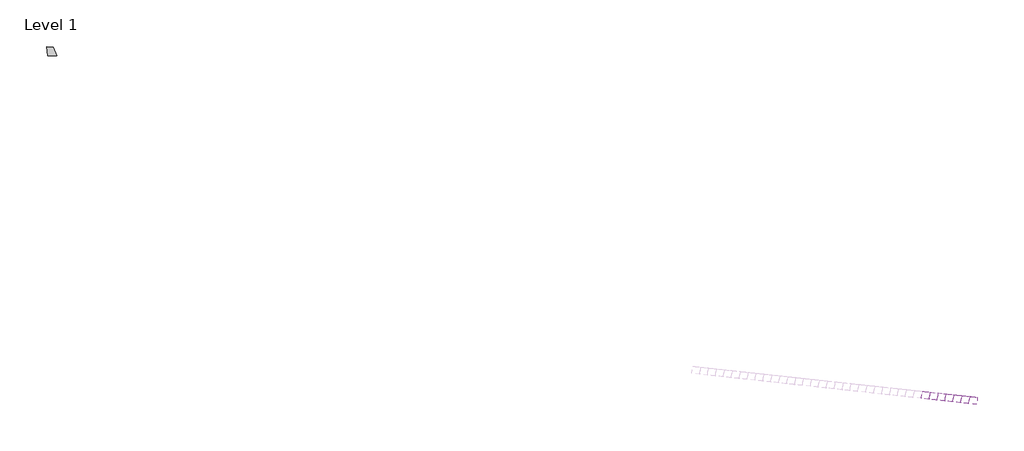
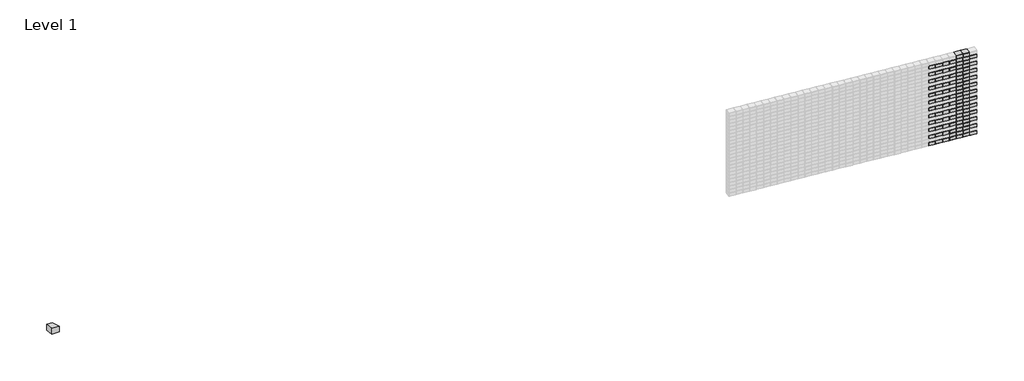
# One storey, part 18 of 18: 111 proxies.
"""IFC4 building model written with IfcOpenShell, lengths in millimetres."""

import ifcopenshell
import ifcopenshell.guid

model = None  # the IFC model being written
_history = None  # IfcOwnerHistory: only IFC2X3 demands one
_inside = {}  # id of a spatial element -> (the spatial element, [elements in it])
_under = {}  # id of a project, library or spatial element -> (it, [spatial elements below it])
_declared = {}  # id of a project -> (the project, [libraries it declares])
_typed = {}  # id of a type object -> (the type object, [elements of that type])
_made_of = {}  # id of a material, layer set ... -> (it, [elements and type objects made of it])


def new_model(schema):
    """Start an empty IFC model of exactly this schema.

    Asked for "IFC4X3", IfcOpenShell would pick the latest addendum, in which some entities
    have other attributes; the version numbers below select the first issue.
    IFC2X3 requires an IfcOwnerHistory on every rooted entity: one is made here for all.
    """
    global model, _history
    if schema == "IFC4X3":
        model = ifcopenshell.file(schema_version=(4, 3, 0, 0))
    else:
        model = ifcopenshell.file(schema=schema)
    _inside.clear()
    _under.clear()
    _declared.clear()
    _typed.clear()
    _made_of.clear()
    _history = None
    if model.schema == "IFC2X3":
        org = make("IfcOrganization", Name="unknown")
        user = make(
            "IfcPersonAndOrganization",
            ThePerson=make("IfcPerson", FamilyName="unknown"),
            TheOrganization=org,
        )
        app = make(
            "IfcApplication",
            ApplicationDeveloper=org,
            Version="unknown",
            ApplicationFullName="unknown",
            ApplicationIdentifier="unknown",
        )
        _history = make(
            "IfcOwnerHistory",
            OwningUser=user,
            OwningApplication=app,
            ChangeAction="ADDED",
            CreationDate=0,
        )
    return model


def make(cls, **values):
    """One entity of the class cls with the attributes given. An attribute that is None is left unset."""
    return model.create_entity(
        cls, **{name: value for name, value in values.items() if value is not None}
    )


def rooted(cls, **values):
    """An entity with a GlobalId (a new one), such as an element, a storey or a relation."""
    return make(cls, GlobalId=ifcopenshell.guid.new(), OwnerHistory=_history, **values)


def si_unit(unit_type, name, prefix=None):
    """IfcSIUnit, for example si_unit("LENGTHUNIT", "METRE", prefix="MILLI")."""
    return make("IfcSIUnit", UnitType=unit_type, Prefix=prefix, Name=name)


def assignment(units):
    """IfcUnitAssignment: the units of a project."""
    return None if units is None else make("IfcUnitAssignment", Units=units)


def point(xyz):
    """IfcCartesianPoint."""
    return None if xyz is None else make("IfcCartesianPoint", Coordinates=xyz)


def direction(xyz):
    """IfcDirection."""
    return None if xyz is None else make("IfcDirection", DirectionRatios=xyz)


def frame(location, z_axis=None, x_axis=None):
    """IfcAxis2Placement3D, a coordinate frame: its origin and axes. An axis left out is left unset."""
    return make(
        "IfcAxis2Placement3D",
        Location=point(location),
        Axis=direction(z_axis),
        RefDirection=direction(x_axis),
    )


def origin():
    """The frame at (0, 0, 0) with its axes left unset."""
    return frame((0.0, 0.0, 0.0))


def origin_with_axes():
    """The frame at (0, 0, 0) with the z axis (0, 0, 1) and the x axis (1, 0, 0) written out."""
    return frame((0.0, 0.0, 0.0), z_axis=(0.0, 0.0, 1.0), x_axis=(1.0, 0.0, 0.0))


def place(relative_to, where):
    """IfcLocalPlacement: puts the frame where relative to a parent placement (None: the world)."""
    return make(
        "IfcLocalPlacement", PlacementRelTo=relative_to, RelativePlacement=where
    )


def context(
    kind, dimensions, precision=None, world=None, true_north=None, identifier=None
):
    """IfcGeometricRepresentationContext, for example the 3D "Model" context."""
    return make(
        "IfcGeometricRepresentationContext",
        ContextIdentifier=identifier,
        ContextType=kind,
        CoordinateSpaceDimension=dimensions,
        Precision=precision,
        WorldCoordinateSystem=world,
        TrueNorth=true_north,
    )


def project(units=None, contexts=None):
    """IfcProject with its units and contexts."""
    return rooted(
        "IfcProject",
        Name="project",
        RepresentationContexts=contexts,
        UnitsInContext=assignment(units),
    )


def spatial(cls, under=None, at=None, **own):
    """A site, building, storey or space (cls), placed at a placement, below another one or the project."""
    s = rooted(cls, ObjectPlacement=at, **own)
    if under is not None:
        _under.setdefault(under.id(), (under, []))[1].append(s)
    return s


def polyline(points):
    """IfcPolyline through the points."""
    return make("IfcPolyline", Points=[point(p) for p in points])


def outline(outer, holes=None, kind="AREA"):
    """IfcArbitraryClosedProfileDef: a profile drawn as a closed curve; with holes, ...WithVoids."""
    if holes is None:
        return make("IfcArbitraryClosedProfileDef", ProfileType=kind, OuterCurve=outer)
    return make(
        "IfcArbitraryProfileDefWithVoids",
        ProfileType=kind,
        OuterCurve=outer,
        InnerCurves=holes,
    )


def extrude(swept, where, along, depth):
    """IfcExtrudedAreaSolid: the profile swept, set in the frame where, extruded along a direction by depth."""
    return make(
        "IfcExtrudedAreaSolid",
        SweptArea=swept,
        Position=where,
        ExtrudedDirection=direction(along),
        Depth=depth,
    )


def shape(context_of_items, identifier, shape_type, items):
    """IfcShapeRepresentation: the items that make up one representation, for example the "Body"."""
    return make(
        "IfcShapeRepresentation",
        ContextOfItems=context_of_items,
        RepresentationIdentifier=identifier,
        RepresentationType=shape_type,
        Items=items,
    )


def source(mapping_origin, context_of_items, identifier, shape_type, items):
    """IfcRepresentationMap: a shape defined once, which mapped items show again and again."""
    return make(
        "IfcRepresentationMap",
        MappingOrigin=mapping_origin,
        MappedRepresentation=shape(context_of_items, identifier, shape_type, items),
    )


def transform(
    local_origin,
    x_axis=None,
    y_axis=None,
    z_axis=None,
    scale=None,
    scale2=None,
    scale3=None,
    uniform=True,
):
    """IfcCartesianTransformationOperator3D, or its non-uniform kind. x_axis, y_axis, z_axis: its Axis1, 2, 3."""
    if uniform:
        return make(
            "IfcCartesianTransformationOperator3D",
            Axis1=direction(x_axis),
            Axis2=direction(y_axis),
            LocalOrigin=point(local_origin),
            Scale=scale,
            Axis3=direction(z_axis),
        )
    return make(
        "IfcCartesianTransformationOperator3DnonUniform",
        Axis1=direction(x_axis),
        Axis2=direction(y_axis),
        LocalOrigin=point(local_origin),
        Scale=scale,
        Axis3=direction(z_axis),
        Scale2=scale2,
        Scale3=scale3,
    )


def mapped(mapping_source, mapping_target):
    """IfcMappedItem: shows the shape of a source again, moved by a transform."""
    return make(
        "IfcMappedItem", MappingSource=mapping_source, MappingTarget=mapping_target
    )


def made_of(thing, what):
    """Note that an element or type object is made of a material, layer set ...; save() writes the relation."""
    if what is not None:
        _made_of.setdefault(what.id(), (what, []))[1].append(thing)
    return thing


def element(
    cls,
    number,
    at=None,
    inside=None,
    cuts=None,
    type_object=None,
    material=None,
    context=None,
    identifier="Body",
    shape_type=None,
    held_by="IfcProductDefinitionShape",
    body=None,
    shapes=None,
    **own,
):
    """One element of the class cls, such as IfcWall. Its Tag is "e" and its number.

    at: its placement. inside: the storey or other place that contains it. cuts: it is an
    opening in that element (IfcRelVoidsElement). A single representation is given by context,
    identifier, shape_type and body (its items); several are given by shapes. held_by: the class
    of the entity that holds the representations. save() writes the other relations.
    """
    e = rooted(cls, Tag="e%d" % number, ObjectPlacement=at, **own)
    if body is not None:
        shapes = [shape(context, identifier, shape_type, body)]
    if shapes is not None:
        e.Representation = make(held_by, Representations=shapes)
    if inside is not None:
        _inside.setdefault(inside.id(), (inside, []))[1].append(e)
    if cuts is not None:
        rooted(
            "IfcRelVoidsElement", RelatingBuildingElement=cuts, RelatedOpeningElement=e
        )
    if type_object is not None:
        _typed.setdefault(type_object.id(), (type_object, []))[1].append(e)
    return made_of(e, material)


def aggregate(whole, parts):
    """IfcRelAggregates: a whole, such as a stair, and the parts it consists of."""
    return rooted("IfcRelAggregates", RelatingObject=whole, RelatedObjects=parts)


def save(model, path):
    """Write the relations noted so far, then the file.

    IfcRelAggregates (storeys below a building ...), IfcRelContainedInSpatialStructure (elements
    in a storey), IfcRelDefinesByType, IfcRelAssociatesMaterial and IfcRelDeclares: one each for
    every whole, place, type object, material and project.
    """
    for whole, parts in _under.values():
        aggregate(whole, parts)
    for where, things in _inside.values():
        rooted(
            "IfcRelContainedInSpatialStructure",
            RelatedElements=things,
            RelatingStructure=where,
        )
    for kind, things in _typed.values():
        rooted("IfcRelDefinesByType", RelatedObjects=things, RelatingType=kind)
    for what, things in _made_of.values():
        rooted("IfcRelAssociatesMaterial", RelatedObjects=things, RelatingMaterial=what)
    for by, libraries in _declared.values():
        rooted("IfcRelDeclares", RelatingContext=by, RelatedDefinitions=libraries)
    model.write(path)


def geel_a5fc7152(model_context):
    return source(origin(), model_context, "Body", "SweptSolid", [
        extrude(outline(polyline([(131.1871262, 51.8695461), (24.8461542, 24.0369432), (23.5801491, 28.8740117), (125.0840527, 55.4406095), (111.9430518, 105.6488784), (10.4391482, 79.0822806), (9.1731432, 83.919349), (115.5141152, 111.7519519), (131.1871262, 51.8695461)])), origin_with_axes(), (0.0, 0.0, 1.0), 95.0),
        extrude(outline(polyline([(111.9430518, 105.6488784), (125.0840527, 55.4406095), (23.5801491, 28.8740117), (10.4391482, 79.0822806), (111.9430518, 105.6488784)])), origin_with_axes(), (0.0, 0.0, 1.0), 100.0),
    ])


def geel_ff5a4212(model_context):
    return source(origin(), model_context, "Body", "SweptSolid", [
        extrude(outline(polyline([(24.8461542, 24.0369432), (9.1731432, 83.919349), (115.5141152, 111.7519519), (116.7801202, 106.9148835), (15.2762167, 80.3482856), (28.4172176, 30.1400167), (129.9211211, 56.7066146), (131.1871262, 51.8695461), (24.8461542, 24.0369432)])), origin_with_axes(), (0.0, 0.0, 1.0), 95.0),
        extrude(outline(polyline([(116.7801202, 106.9148835), (129.9211211, 56.7066146), (28.4172176, 30.1400167), (15.2762167, 80.3482856), (116.7801202, 106.9148835)])), origin_with_axes(), (0.0, 0.0, 1.0), 100.0),
    ])


def rood_14a66368(model_context):
    return source(origin(), model_context, "Body", "SweptSolid", [
        extrude(outline(polyline([(24.8461542, 24.0369432), (9.1731432, 83.919349), (115.5141152, 111.7519519), (131.1871262, 51.8695461), (24.8461542, 24.0369432)]), holes=[polyline([(125.0840527, 55.4406095), (111.9430518, 105.6488784), (15.2762167, 80.3482856), (28.4172176, 30.1400167), (125.0840527, 55.4406095)])]), origin_with_axes(), (0.0, 0.0, 1.0), 95.0),
        extrude(outline(polyline([(111.9430518, 105.6488784), (125.0840527, 55.4406095), (28.4172176, 30.1400167), (15.2762167, 80.3482856), (111.9430518, 105.6488784)])), origin_with_axes(), (0.0, 0.0, 1.0), 100.0),
    ])


def rood_2ddd8018(model_context):
    return source(origin(), model_context, "Body", "SweptSolid", [
        extrude(outline(polyline([(24.8461542, 24.0369432), (9.1731432, 83.919349), (115.5141152, 111.7519519), (131.1871262, 51.8695461), (126.3500577, 50.6035411), (111.9430518, 105.6488784), (15.2762167, 80.3482856), (29.6832226, 25.3029482), (24.8461542, 24.0369432)])), origin_with_axes(), (0.0, 0.0, 1.0), 95.0),
        extrude(outline(polyline([(111.9430518, 105.6488784), (126.3500577, 50.6035411), (29.6832226, 25.3029482), (15.2762167, 80.3482856), (111.9430518, 105.6488784)])), origin_with_axes(), (0.0, 0.0, 1.0), 100.0),
    ])


def steen_standaard_rood_a5b9f397(model_context):
    return source(origin(), model_context, "Body", "SweptSolid", [
        extrude(outline(polyline([(82.4636514, 127.1543377), (128.4615135, 4.6891223), (4.3616271, 4.9486265), (-12.4180967, 134.7857038), (82.4636514, 127.1543377)])), origin_with_axes(), (0.0, 0.0, 1.0), 100.0),
    ])


model = new_model("IFC4")

# Units and contexts
model_context = context("Model", 3, world=origin())
ifc_project = project(units=[si_unit("LENGTHUNIT", "METRE", prefix="MILLI")], contexts=[model_context])

# Site, building, storey
site = spatial("IfcSite", under=ifc_project)
building = spatial("IfcBuilding", under=site)
storey = spatial("IfcBuildingStorey", under=building, Name="Level 1", Elevation=0.0)

# Proxies
placement = place(None, origin())
geel_shape = geel_a5fc7152(model_context)
element("IfcBuildingElementProxy", 1, Name="Geel", ObjectType="Geel", at=placement, inside=storey, context=model_context, shape_type="MappedRepresentation", body=[
    mapped(geel_shape, transform((12373.9492488, -4657.0823366, 2044.9368847), x_axis=(0.961727550372943, -0.10473475661477032, -0.25320100633785686), y_axis=(0.25171277368867245, -0.02741220845642687, 0.9674136914420308), z_axis=(-0.10826263628608798, -0.9941223272738553, 0.0))),
])
element("IfcBuildingElementProxy", 2, Name="Geel", ObjectType="Geel", at=placement, inside=storey, context=model_context, shape_type="MappedRepresentation", body=[
    mapped(geel_shape, transform((12592.5029772, -4680.8834345, 2168.7358475), x_axis=(0.9617275503729374, -0.1047347566147725, -0.25320100633787673), y_axis=(0.25171277368869216, -0.02741220845642974, 0.9674136914420255), z_axis=(-0.10826263628609081, -0.9941223272738551, 0.0))),
])
element("IfcBuildingElementProxy", 3, Name="Geel", ObjectType="Geel", at=placement, inside=storey, context=model_context, shape_type="MappedRepresentation", body=[
    mapped(geel_shape, transform((12592.5029772, -4680.8834345, 2292.5348104), x_axis=(0.9617275503729374, -0.1047347566147725, -0.25320100633787673), y_axis=(0.25171277368869216, -0.02741220845642974, 0.9674136914420255), z_axis=(-0.10826263628609081, -0.9941223272738551, 0.0))),
])
element("IfcBuildingElementProxy", 4, Name="Geel", ObjectType="Geel", at=placement, inside=storey, context=model_context, shape_type="MappedRepresentation", body=[
    mapped(geel_shape, transform((12592.5029772, -4680.8834345, 2416.3337732), x_axis=(0.9617275503729384, -0.1047347566147726, -0.25320100633787307), y_axis=(0.25171277368868855, -0.02741220845642934, 0.9674136914420265), z_axis=(-0.10826263628609081, -0.994122327273855, 0.0))),
])
element("IfcBuildingElementProxy", 5, Name="Geel", ObjectType="Geel", at=placement, inside=storey, context=model_context, shape_type="MappedRepresentation", body=[
    mapped(geel_shape, transform((12592.5029772, -4680.8834345, 2540.132736), x_axis=(0.9617275503729374, -0.1047347566147725, -0.25320100633787673), y_axis=(0.25171277368869216, -0.02741220845642974, 0.9674136914420255), z_axis=(-0.10826263628609081, -0.9941223272738551, 0.0))),
])
element("IfcBuildingElementProxy", 6, Name="Geel", ObjectType="Geel", at=placement, inside=storey, context=model_context, shape_type="MappedRepresentation", body=[
    mapped(geel_shape, transform((12592.5029772, -4680.8834345, 2663.9316989), x_axis=(0.9617275503729374, -0.1047347566147725, -0.25320100633787673), y_axis=(0.25171277368869216, -0.02741220845642974, 0.9674136914420255), z_axis=(-0.10826263628609081, -0.9941223272738551, 0.0))),
])
element("IfcBuildingElementProxy", 7, Name="Geel", ObjectType="Geel", at=placement, inside=storey, context=model_context, shape_type="MappedRepresentation", body=[
    mapped(geel_shape, transform((12592.5029772, -4680.8834345, 2787.7306617), x_axis=(0.9617275503729374, -0.1047347566147725, -0.25320100633787673), y_axis=(0.25171277368869216, -0.02741220845642974, 0.9674136914420255), z_axis=(-0.10826263628609081, -0.9941223272738551, 0.0))),
])
element("IfcBuildingElementProxy", 8, Name="Geel", ObjectType="Geel", at=placement, inside=storey, context=model_context, shape_type="MappedRepresentation", body=[
    mapped(geel_shape, transform((12592.5029772, -4680.8834345, 2911.5296245), x_axis=(0.9617275503729374, -0.1047347566147725, -0.25320100633787673), y_axis=(0.25171277368869216, -0.02741220845642974, 0.9674136914420255), z_axis=(-0.10826263628609081, -0.9941223272738551, 0.0))),
])
element("IfcBuildingElementProxy", 9, Name="Geel", ObjectType="Geel", at=placement, inside=storey, context=model_context, shape_type="MappedRepresentation", body=[
    mapped(geel_shape, transform((12592.5029772, -4680.8834345, 3035.3285874), x_axis=(0.9617275503729374, -0.1047347566147725, -0.25320100633787673), y_axis=(0.25171277368869216, -0.02741220845642974, 0.9674136914420255), z_axis=(-0.10826263628609081, -0.9941223272738551, 0.0))),
])
element("IfcBuildingElementProxy", 10, Name="Geel", ObjectType="Geel", at=placement, inside=storey, context=model_context, shape_type="MappedRepresentation", body=[
    mapped(geel_shape, transform((12592.5029772, -4680.8834345, 3159.1275502), x_axis=(0.9617275503729374, -0.1047347566147725, -0.25320100633787673), y_axis=(0.25171277368869216, -0.02741220845642974, 0.9674136914420255), z_axis=(-0.10826263628609081, -0.9941223272738551, 0.0))),
])
element("IfcBuildingElementProxy", 11, Name="Geel", ObjectType="Geel", at=placement, inside=storey, context=model_context, shape_type="MappedRepresentation", body=[
    mapped(geel_shape, transform((12592.5029772, -4680.8834345, 3282.926513), x_axis=(0.9617275503729374, -0.1047347566147725, -0.25320100633787673), y_axis=(0.25171277368869216, -0.02741220845642974, 0.9674136914420255), z_axis=(-0.10826263628609081, -0.9941223272738551, 0.0))),
])
element("IfcBuildingElementProxy", 12, Name="Geel", ObjectType="Geel", at=placement, inside=storey, context=model_context, shape_type="MappedRepresentation", body=[
    mapped(geel_shape, transform((12592.5029772, -4680.8834345, 3406.7254759), x_axis=(0.9617275503729374, -0.1047347566147725, -0.25320100633787673), y_axis=(0.25171277368869216, -0.02741220845642974, 0.9674136914420255), z_axis=(-0.10826263628609081, -0.9941223272738551, 0.0))),
])
element("IfcBuildingElementProxy", 13, Name="Geel", ObjectType="Geel", at=placement, inside=storey, context=model_context, shape_type="MappedRepresentation", body=[
    mapped(geel_shape, transform((12592.5029772, -4680.8834345, 2044.9368847), x_axis=(0.9617275503729384, -0.1047347566147726, -0.25320100633787307), y_axis=(0.25171277368868855, -0.02741220845642934, 0.9674136914420265), z_axis=(-0.10826263628609081, -0.994122327273855, 0.0))),
])
geel_2_shape = geel_ff5a4212(model_context)
element("IfcBuildingElementProxy", 14, Name="Geel", ObjectType="Geel", at=placement, inside=storey, context=model_context, shape_type="MappedRepresentation", body=[
    mapped(geel_2_shape, transform((12483.226113, -4668.9828856, 2168.7358475), x_axis=(0.9617275503729374, -0.1047347566147725, -0.25320100633787673), y_axis=(0.25171277368869216, -0.02741220845642974, 0.9674136914420255), z_axis=(-0.10826263628609081, -0.9941223272738551, 0.0))),
])
element("IfcBuildingElementProxy", 15, Name="Geel", ObjectType="Geel", at=placement, inside=storey, context=model_context, shape_type="MappedRepresentation", body=[
    mapped(geel_2_shape, transform((12483.226113, -4668.9828856, 2292.5348104), x_axis=(0.9617275503729374, -0.1047347566147725, -0.25320100633787673), y_axis=(0.25171277368869216, -0.02741220845642974, 0.9674136914420255), z_axis=(-0.10826263628609081, -0.9941223272738551, 0.0))),
])
element("IfcBuildingElementProxy", 16, Name="Geel", ObjectType="Geel", at=placement, inside=storey, context=model_context, shape_type="MappedRepresentation", body=[
    mapped(geel_2_shape, transform((12483.226113, -4668.9828856, 2416.3337732), x_axis=(0.9617275503729384, -0.1047347566147726, -0.25320100633787307), y_axis=(0.25171277368868855, -0.02741220845642934, 0.9674136914420265), z_axis=(-0.10826263628609081, -0.994122327273855, 0.0))),
])
element("IfcBuildingElementProxy", 17, Name="Geel", ObjectType="Geel", at=placement, inside=storey, context=model_context, shape_type="MappedRepresentation", body=[
    mapped(geel_2_shape, transform((12483.226113, -4668.9828856, 2540.132736), x_axis=(0.9617275503729374, -0.1047347566147725, -0.25320100633787673), y_axis=(0.25171277368869216, -0.02741220845642974, 0.9674136914420255), z_axis=(-0.10826263628609081, -0.9941223272738551, 0.0))),
])
element("IfcBuildingElementProxy", 18, Name="Geel", ObjectType="Geel", at=placement, inside=storey, context=model_context, shape_type="MappedRepresentation", body=[
    mapped(geel_2_shape, transform((12483.226113, -4668.9828856, 2663.9316989), x_axis=(0.9617275503729374, -0.1047347566147725, -0.25320100633787673), y_axis=(0.25171277368869216, -0.02741220845642974, 0.9674136914420255), z_axis=(-0.10826263628609081, -0.9941223272738551, 0.0))),
])
element("IfcBuildingElementProxy", 19, Name="Geel", ObjectType="Geel", at=placement, inside=storey, context=model_context, shape_type="MappedRepresentation", body=[
    mapped(geel_2_shape, transform((12483.226113, -4668.9828856, 2787.7306617), x_axis=(0.9617275503729374, -0.1047347566147725, -0.25320100633787673), y_axis=(0.25171277368869216, -0.02741220845642974, 0.9674136914420255), z_axis=(-0.10826263628609081, -0.9941223272738551, 0.0))),
])
element("IfcBuildingElementProxy", 20, Name="Geel", ObjectType="Geel", at=placement, inside=storey, context=model_context, shape_type="MappedRepresentation", body=[
    mapped(geel_2_shape, transform((12483.226113, -4668.9828856, 2911.5296245), x_axis=(0.9617275503729374, -0.1047347566147725, -0.25320100633787673), y_axis=(0.25171277368869216, -0.02741220845642974, 0.9674136914420255), z_axis=(-0.10826263628609081, -0.9941223272738551, 0.0))),
])
element("IfcBuildingElementProxy", 21, Name="Geel", ObjectType="Geel", at=placement, inside=storey, context=model_context, shape_type="MappedRepresentation", body=[
    mapped(geel_2_shape, transform((12483.226113, -4668.9828856, 3035.3285874), x_axis=(0.9617275503729374, -0.1047347566147725, -0.25320100633787673), y_axis=(0.25171277368869216, -0.02741220845642974, 0.9674136914420255), z_axis=(-0.10826263628609081, -0.9941223272738551, 0.0))),
])
element("IfcBuildingElementProxy", 22, Name="Geel", ObjectType="Geel", at=placement, inside=storey, context=model_context, shape_type="MappedRepresentation", body=[
    mapped(geel_2_shape, transform((12483.226113, -4668.9828856, 3159.1275502), x_axis=(0.9617275503729374, -0.1047347566147725, -0.25320100633787673), y_axis=(0.25171277368869216, -0.02741220845642974, 0.9674136914420255), z_axis=(-0.10826263628609081, -0.9941223272738551, 0.0))),
])
element("IfcBuildingElementProxy", 23, Name="Geel", ObjectType="Geel", at=placement, inside=storey, context=model_context, shape_type="MappedRepresentation", body=[
    mapped(geel_2_shape, transform((12483.226113, -4668.9828856, 3282.926513), x_axis=(0.9617275503729374, -0.1047347566147725, -0.25320100633787673), y_axis=(0.25171277368869216, -0.02741220845642974, 0.9674136914420255), z_axis=(-0.10826263628609081, -0.9941223272738551, 0.0))),
])
element("IfcBuildingElementProxy", 24, Name="Geel", ObjectType="Geel", at=placement, inside=storey, context=model_context, shape_type="MappedRepresentation", body=[
    mapped(geel_2_shape, transform((12483.226113, -4668.9828856, 3406.7254759), x_axis=(0.9617275503729374, -0.1047347566147725, -0.25320100633787673), y_axis=(0.25171277368869216, -0.02741220845642974, 0.9674136914420255), z_axis=(-0.10826263628609081, -0.9941223272738551, 0.0))),
])
element("IfcBuildingElementProxy", 25, Name="Geel", ObjectType="Geel", at=placement, inside=storey, context=model_context, shape_type="MappedRepresentation", body=[
    mapped(geel_2_shape, transform((12483.226113, -4668.9828856, 2044.9368847), x_axis=(0.9617275503729384, -0.1047347566147726, -0.25320100633787307), y_axis=(0.25171277368868855, -0.02741220845642934, 0.9674136914420265), z_axis=(-0.10826263628609081, -0.994122327273855, 0.0))),
])
element("IfcBuildingElementProxy", 26, Name="Rood", ObjectType="Rood", at=placement, inside=storey, context=model_context, shape_type="MappedRepresentation", body=[
    mapped(geel_shape, transform((12701.7798414, -4692.7839834, 2106.8363661), x_axis=(0.9617275503729374, -0.1047347566147725, -0.25320100633787673), y_axis=(0.25171277368869216, -0.02741220845642974, 0.9674136914420255), z_axis=(-0.10826263628609081, -0.9941223272738551, 0.0))),
])
element("IfcBuildingElementProxy", 27, Name="Rood", ObjectType="Rood", at=placement, inside=storey, context=model_context, shape_type="MappedRepresentation", body=[
    mapped(geel_shape, transform((12701.7798414, -4692.7839834, 2230.6353289), x_axis=(0.9617275503729384, -0.1047347566147726, -0.25320100633787307), y_axis=(0.25171277368868855, -0.02741220845642934, 0.9674136914420265), z_axis=(-0.10826263628609081, -0.994122327273855, 0.0))),
])
element("IfcBuildingElementProxy", 28, Name="Rood", ObjectType="Rood", at=placement, inside=storey, context=model_context, shape_type="MappedRepresentation", body=[
    mapped(geel_shape, transform((12701.7798414, -4692.7839834, 2354.4342918), x_axis=(0.9617275503729374, -0.1047347566147725, -0.25320100633787673), y_axis=(0.25171277368869216, -0.02741220845642974, 0.9674136914420255), z_axis=(-0.10826263628609081, -0.9941223272738551, 0.0))),
])
element("IfcBuildingElementProxy", 29, Name="Rood", ObjectType="Rood", at=placement, inside=storey, context=model_context, shape_type="MappedRepresentation", body=[
    mapped(geel_shape, transform((12701.7798414, -4692.7839834, 2478.2332546), x_axis=(0.9617275503729374, -0.1047347566147725, -0.25320100633787673), y_axis=(0.25171277368869216, -0.02741220845642974, 0.9674136914420255), z_axis=(-0.10826263628609081, -0.9941223272738551, 0.0))),
])
element("IfcBuildingElementProxy", 30, Name="Rood", ObjectType="Rood", at=placement, inside=storey, context=model_context, shape_type="MappedRepresentation", body=[
    mapped(geel_shape, transform((12701.7798414, -4692.7839834, 2602.0322174), x_axis=(0.9617275503729394, -0.10473475661477268, -0.2532010063378695), y_axis=(0.2517127736886849, -0.027412208456428923, 0.9674136914420275), z_axis=(-0.1082626362860908, -0.9941223272738551, 0.0))),
])
element("IfcBuildingElementProxy", 31, Name="Rood", ObjectType="Rood", at=placement, inside=storey, context=model_context, shape_type="MappedRepresentation", body=[
    mapped(geel_shape, transform((12701.7798414, -4692.7839834, 2725.8311803), x_axis=(0.9617275503729374, -0.1047347566147725, -0.25320100633787673), y_axis=(0.25171277368869216, -0.02741220845642974, 0.9674136914420255), z_axis=(-0.10826263628609081, -0.9941223272738551, 0.0))),
])
element("IfcBuildingElementProxy", 32, Name="Rood", ObjectType="Rood", at=placement, inside=storey, context=model_context, shape_type="MappedRepresentation", body=[
    mapped(geel_shape, transform((12701.7798414, -4692.7839834, 2849.6301431), x_axis=(0.9617275503729374, -0.1047347566147725, -0.25320100633787673), y_axis=(0.25171277368869216, -0.02741220845642974, 0.9674136914420255), z_axis=(-0.10826263628609081, -0.9941223272738551, 0.0))),
])
element("IfcBuildingElementProxy", 33, Name="Rood", ObjectType="Rood", at=placement, inside=storey, context=model_context, shape_type="MappedRepresentation", body=[
    mapped(geel_shape, transform((12701.7798414, -4692.7839834, 2973.4291059), x_axis=(0.9617275503729374, -0.1047347566147725, -0.25320100633787673), y_axis=(0.25171277368869216, -0.02741220845642974, 0.9674136914420255), z_axis=(-0.10826263628609081, -0.9941223272738551, 0.0))),
])
element("IfcBuildingElementProxy", 34, Name="Rood", ObjectType="Rood", at=placement, inside=storey, context=model_context, shape_type="MappedRepresentation", body=[
    mapped(geel_shape, transform((12701.7798414, -4692.7839834, 3097.2280688), x_axis=(0.9617275503729394, -0.10473475661477268, -0.2532010063378695), y_axis=(0.2517127736886849, -0.027412208456428923, 0.9674136914420275), z_axis=(-0.1082626362860908, -0.9941223272738551, 0.0))),
])
element("IfcBuildingElementProxy", 35, Name="Rood", ObjectType="Rood", at=placement, inside=storey, context=model_context, shape_type="MappedRepresentation", body=[
    mapped(geel_shape, transform((12701.7798414, -4692.7839834, 3221.0270316), x_axis=(0.9617275503729374, -0.1047347566147725, -0.25320100633787673), y_axis=(0.25171277368869216, -0.02741220845642974, 0.9674136914420255), z_axis=(-0.10826263628609081, -0.9941223272738551, 0.0))),
])
element("IfcBuildingElementProxy", 36, Name="Rood", ObjectType="Rood", at=placement, inside=storey, context=model_context, shape_type="MappedRepresentation", body=[
    mapped(geel_shape, transform((12701.7798414, -4692.7839834, 3344.8259944), x_axis=(0.9617275503729357, -0.10473475661477229, -0.2532010063378841), y_axis=(0.2517127736886993, -0.027412208456430498, 0.9674136914420237), z_axis=(-0.10826263628609081, -0.9941223272738551, 0.0))),
])
element("IfcBuildingElementProxy", 37, Name="Rood", ObjectType="Rood", at=placement, inside=storey, context=model_context, shape_type="MappedRepresentation", body=[
    mapped(geel_shape, transform((12701.7798414, -4692.7839834, 1983.0374033), x_axis=(0.9617275503729374, -0.1047347566147725, -0.25320100633787673), y_axis=(0.25171277368869216, -0.02741220845642974, 0.9674136914420255), z_axis=(-0.10826263628609081, -0.9941223272738551, 0.0))),
])
rood_shape = rood_14a66368(model_context)
element("IfcBuildingElementProxy", 38, Name="Rood", ObjectType="Rood", at=placement, inside=storey, context=model_context, shape_type="MappedRepresentation", body=[
    mapped(rood_shape, transform((12046.1186563, -4621.3806898, 2106.8363661), x_axis=(0.9617275503729374, -0.10473475661477244, -0.25320100633787673), y_axis=(0.25171277368869216, -0.02741220845642972, 0.9674136914420255), z_axis=(-0.10826263628609079, -0.9941223272738551, 0.0))),
])
element("IfcBuildingElementProxy", 39, Name="Rood", ObjectType="Rood", at=placement, inside=storey, context=model_context, shape_type="MappedRepresentation", body=[
    mapped(rood_shape, transform((12046.1186563, -4621.3806898, 2230.6353289), x_axis=(0.9617275503729384, -0.10473475661477256, -0.25320100633787307), y_axis=(0.25171277368868855, -0.02741220845642932, 0.9674136914420265), z_axis=(-0.10826263628609077, -0.994122327273855, 0.0))),
])
element("IfcBuildingElementProxy", 40, Name="Rood", ObjectType="Rood", at=placement, inside=storey, context=model_context, shape_type="MappedRepresentation", body=[
    mapped(rood_shape, transform((12046.1186563, -4621.3806898, 2354.4342918), x_axis=(0.9617275503729374, -0.10473475661477244, -0.25320100633787673), y_axis=(0.25171277368869216, -0.02741220845642972, 0.9674136914420255), z_axis=(-0.10826263628609079, -0.9941223272738551, 0.0))),
])
element("IfcBuildingElementProxy", 41, Name="Rood", ObjectType="Rood", at=placement, inside=storey, context=model_context, shape_type="MappedRepresentation", body=[
    mapped(rood_shape, transform((12046.1186563, -4621.3806898, 2478.2332546), x_axis=(0.9617275503729374, -0.10473475661477244, -0.25320100633787673), y_axis=(0.25171277368869216, -0.02741220845642972, 0.9674136914420255), z_axis=(-0.10826263628609079, -0.9941223272738551, 0.0))),
])
element("IfcBuildingElementProxy", 42, Name="Rood", ObjectType="Rood", at=placement, inside=storey, context=model_context, shape_type="MappedRepresentation", body=[
    mapped(rood_shape, transform((12046.1186563, -4621.3806898, 2602.0322174), x_axis=(0.9617275503729394, -0.10473475661477263, -0.2532010063378695), y_axis=(0.2517127736886849, -0.027412208456428916, 0.9674136914420275), z_axis=(-0.10826263628609077, -0.9941223272738551, 0.0))),
])
element("IfcBuildingElementProxy", 43, Name="Rood", ObjectType="Rood", at=placement, inside=storey, context=model_context, shape_type="MappedRepresentation", body=[
    mapped(rood_shape, transform((12046.1186563, -4621.3806898, 2725.8311803), x_axis=(0.9617275503729374, -0.10473475661477244, -0.25320100633787673), y_axis=(0.25171277368869216, -0.02741220845642972, 0.9674136914420255), z_axis=(-0.10826263628609079, -0.9941223272738551, 0.0))),
])
element("IfcBuildingElementProxy", 44, Name="Rood", ObjectType="Rood", at=placement, inside=storey, context=model_context, shape_type="MappedRepresentation", body=[
    mapped(rood_shape, transform((12046.1186563, -4621.3806898, 2849.6301431), x_axis=(0.9617275503729374, -0.10473475661477244, -0.25320100633787673), y_axis=(0.25171277368869216, -0.02741220845642972, 0.9674136914420255), z_axis=(-0.10826263628609079, -0.9941223272738551, 0.0))),
])
element("IfcBuildingElementProxy", 45, Name="Rood", ObjectType="Rood", at=placement, inside=storey, context=model_context, shape_type="MappedRepresentation", body=[
    mapped(rood_shape, transform((12046.1186563, -4621.3806898, 2973.4291059), x_axis=(0.9617275503729374, -0.10473475661477244, -0.25320100633787673), y_axis=(0.25171277368869216, -0.02741220845642972, 0.9674136914420255), z_axis=(-0.10826263628609079, -0.9941223272738551, 0.0))),
])
element("IfcBuildingElementProxy", 46, Name="Rood", ObjectType="Rood", at=placement, inside=storey, context=model_context, shape_type="MappedRepresentation", body=[
    mapped(rood_shape, transform((12046.1186563, -4621.3806898, 3097.2280688), x_axis=(0.9617275503729394, -0.10473475661477263, -0.2532010063378695), y_axis=(0.2517127736886849, -0.027412208456428916, 0.9674136914420275), z_axis=(-0.10826263628609077, -0.9941223272738551, 0.0))),
])
element("IfcBuildingElementProxy", 47, Name="Rood", ObjectType="Rood", at=placement, inside=storey, context=model_context, shape_type="MappedRepresentation", body=[
    mapped(rood_shape, transform((12046.1186563, -4621.3806898, 3221.0270316), x_axis=(0.9617275503729374, -0.10473475661477244, -0.25320100633787673), y_axis=(0.25171277368869216, -0.02741220845642972, 0.9674136914420255), z_axis=(-0.10826263628609079, -0.9941223272738551, 0.0))),
])
element("IfcBuildingElementProxy", 48, Name="Rood", ObjectType="Rood", at=placement, inside=storey, context=model_context, shape_type="MappedRepresentation", body=[
    mapped(rood_shape, transform((12046.1186563, -4621.3806898, 3344.8259944), x_axis=(0.9617275503729357, -0.10473475661477225, -0.2532010063378841), y_axis=(0.2517127736886993, -0.027412208456430477, 0.9674136914420237), z_axis=(-0.10826263628609077, -0.9941223272738551, 0.0))),
])
element("IfcBuildingElementProxy", 49, Name="Rood", ObjectType="Rood", at=placement, inside=storey, context=model_context, shape_type="MappedRepresentation", body=[
    mapped(rood_shape, transform((12046.1186563, -4621.3806898, 1983.0374033), x_axis=(0.9617275503729374, -0.10473475661477244, -0.25320100633787673), y_axis=(0.25171277368869216, -0.02741220845642972, 0.9674136914420255), z_axis=(-0.10826263628609079, -0.9941223272738551, 0.0))),
])
element("IfcBuildingElementProxy", 50, Name="Rood", ObjectType="Rood", at=placement, inside=storey, context=model_context, shape_type="MappedRepresentation", body=[
    mapped(rood_shape, transform((12155.3955205, -4633.2812388, 2106.8363661), x_axis=(0.9617275503729422, -0.10473475661477022, -0.25320100633786), y_axis=(0.25171277368867573, -0.02741220845642721, 0.9674136914420299), z_axis=(-0.10826263628608798, -0.9941223272738554, 0.0))),
])
element("IfcBuildingElementProxy", 51, Name="Rood", ObjectType="Rood", at=placement, inside=storey, context=model_context, shape_type="MappedRepresentation", body=[
    mapped(rood_shape, transform((12155.3955205, -4633.2812388, 2230.6353289), x_axis=(0.961727550372943, -0.10473475661477033, -0.25320100633785647), y_axis=(0.25171277368867206, -0.0274122084564268, 0.9674136914420309), z_axis=(-0.10826263628608797, -0.9941223272738553, 0.0))),
])
element("IfcBuildingElementProxy", 52, Name="Rood", ObjectType="Rood", at=placement, inside=storey, context=model_context, shape_type="MappedRepresentation", body=[
    mapped(rood_shape, transform((12155.3955205, -4633.2812388, 2354.4342918), x_axis=(0.9617275503729422, -0.10473475661477022, -0.25320100633786), y_axis=(0.25171277368867573, -0.02741220845642721, 0.9674136914420299), z_axis=(-0.10826263628608798, -0.9941223272738554, 0.0))),
])
element("IfcBuildingElementProxy", 53, Name="Rood", ObjectType="Rood", at=placement, inside=storey, context=model_context, shape_type="MappedRepresentation", body=[
    mapped(rood_shape, transform((12155.3955205, -4633.2812388, 2478.2332546), x_axis=(0.9617275503729422, -0.10473475661477022, -0.25320100633786), y_axis=(0.25171277368867573, -0.02741220845642721, 0.9674136914420299), z_axis=(-0.10826263628608798, -0.9941223272738554, 0.0))),
])
element("IfcBuildingElementProxy", 54, Name="Rood", ObjectType="Rood", at=placement, inside=storey, context=model_context, shape_type="MappedRepresentation", body=[
    mapped(rood_shape, transform((12155.3955205, -4633.2812388, 2602.0322174), x_axis=(0.9617275503729441, -0.10473475661477044, -0.2532010063378528), y_axis=(0.2517127736886685, -0.027412208456426425, 0.9674136914420318), z_axis=(-0.10826263628608798, -0.9941223272738553, 0.0))),
])
element("IfcBuildingElementProxy", 55, Name="Rood", ObjectType="Rood", at=placement, inside=storey, context=model_context, shape_type="MappedRepresentation", body=[
    mapped(rood_shape, transform((12155.3955205, -4633.2812388, 2725.8311803), x_axis=(0.9617275503729422, -0.10473475661477022, -0.25320100633786), y_axis=(0.25171277368867573, -0.02741220845642721, 0.9674136914420299), z_axis=(-0.10826263628608798, -0.9941223272738554, 0.0))),
])
element("IfcBuildingElementProxy", 56, Name="Rood", ObjectType="Rood", at=placement, inside=storey, context=model_context, shape_type="MappedRepresentation", body=[
    mapped(rood_shape, transform((12155.3955205, -4633.2812388, 2849.6301431), x_axis=(0.9617275503729422, -0.10473475661477022, -0.25320100633786), y_axis=(0.25171277368867573, -0.02741220845642721, 0.9674136914420299), z_axis=(-0.10826263628608798, -0.9941223272738554, 0.0))),
])
element("IfcBuildingElementProxy", 57, Name="Rood", ObjectType="Rood", at=placement, inside=storey, context=model_context, shape_type="MappedRepresentation", body=[
    mapped(rood_shape, transform((12155.3955205, -4633.2812388, 2973.4291059), x_axis=(0.9617275503729422, -0.10473475661477022, -0.25320100633786), y_axis=(0.25171277368867573, -0.02741220845642721, 0.9674136914420299), z_axis=(-0.10826263628608798, -0.9941223272738554, 0.0))),
])
element("IfcBuildingElementProxy", 58, Name="Rood", ObjectType="Rood", at=placement, inside=storey, context=model_context, shape_type="MappedRepresentation", body=[
    mapped(rood_shape, transform((12155.3955205, -4633.2812388, 3097.2280688), x_axis=(0.9617275503729441, -0.10473475661477044, -0.2532010063378528), y_axis=(0.2517127736886685, -0.027412208456426425, 0.9674136914420318), z_axis=(-0.10826263628608798, -0.9941223272738553, 0.0))),
])
element("IfcBuildingElementProxy", 59, Name="Rood", ObjectType="Rood", at=placement, inside=storey, context=model_context, shape_type="MappedRepresentation", body=[
    mapped(rood_shape, transform((12155.3955205, -4633.2812388, 3221.0270316), x_axis=(0.9617275503729422, -0.10473475661477022, -0.25320100633786), y_axis=(0.25171277368867573, -0.02741220845642721, 0.9674136914420299), z_axis=(-0.10826263628608798, -0.9941223272738554, 0.0))),
])
element("IfcBuildingElementProxy", 60, Name="Rood", ObjectType="Rood", at=placement, inside=storey, context=model_context, shape_type="MappedRepresentation", body=[
    mapped(rood_shape, transform((12155.3955205, -4633.2812388, 3344.8259944), x_axis=(0.9617275503729402, -0.10473475661477001, -0.2532010063378673), y_axis=(0.25171277368868267, -0.027412208456427965, 0.9674136914420282), z_axis=(-0.10826263628608797, -0.9941223272738553, 0.0))),
])
element("IfcBuildingElementProxy", 61, Name="Rood", ObjectType="Rood", at=placement, inside=storey, context=model_context, shape_type="MappedRepresentation", body=[
    mapped(rood_shape, transform((12155.3955205, -4633.2812388, 1983.0374033), x_axis=(0.9617275503729422, -0.10473475661477022, -0.25320100633786), y_axis=(0.25171277368867573, -0.02741220845642721, 0.9674136914420299), z_axis=(-0.10826263628608798, -0.9941223272738554, 0.0))),
])
element("IfcBuildingElementProxy", 62, Name="Rood", ObjectType="Rood", at=placement, inside=storey, context=model_context, shape_type="MappedRepresentation", body=[
    mapped(rood_shape, transform((12373.9492488, -4657.0823366, 2106.8363661), x_axis=(0.961727550372942, -0.1047347566147702, -0.25320100633786047), y_axis=(0.2517127736886762, -0.02741220845642727, 0.9674136914420297), z_axis=(-0.10826263628608798, -0.9941223272738554, 0.0))),
])
element("IfcBuildingElementProxy", 63, Name="Rood", ObjectType="Rood", at=placement, inside=storey, context=model_context, shape_type="MappedRepresentation", body=[
    mapped(rood_shape, transform((12373.9492488, -4657.0823366, 2230.6353289), x_axis=(0.961727550372943, -0.10473475661477032, -0.25320100633785686), y_axis=(0.25171277368867245, -0.02741220845642687, 0.9674136914420308), z_axis=(-0.10826263628608798, -0.9941223272738553, 0.0))),
])
element("IfcBuildingElementProxy", 64, Name="Rood", ObjectType="Rood", at=placement, inside=storey, context=model_context, shape_type="MappedRepresentation", body=[
    mapped(rood_shape, transform((12373.9492488, -4657.0823366, 2354.4342918), x_axis=(0.961727550372942, -0.1047347566147702, -0.25320100633786047), y_axis=(0.2517127736886762, -0.02741220845642727, 0.9674136914420297), z_axis=(-0.10826263628608798, -0.9941223272738554, 0.0))),
])
element("IfcBuildingElementProxy", 65, Name="Rood", ObjectType="Rood", at=placement, inside=storey, context=model_context, shape_type="MappedRepresentation", body=[
    mapped(rood_shape, transform((12373.9492488, -4657.0823366, 2478.2332546), x_axis=(0.961727550372942, -0.1047347566147702, -0.25320100633786047), y_axis=(0.2517127736886762, -0.02741220845642727, 0.9674136914420297), z_axis=(-0.10826263628608798, -0.9941223272738554, 0.0))),
])
element("IfcBuildingElementProxy", 66, Name="Rood", ObjectType="Rood", at=placement, inside=storey, context=model_context, shape_type="MappedRepresentation", body=[
    mapped(rood_shape, transform((12373.9492488, -4657.0823366, 2602.0322174), x_axis=(0.9617275503729439, -0.10473475661477041, -0.2532010063378535), y_axis=(0.2517127736886689, -0.027412208456426453, 0.9674136914420317), z_axis=(-0.10826263628608798, -0.9941223272738554, 0.0))),
])
element("IfcBuildingElementProxy", 67, Name="Rood", ObjectType="Rood", at=placement, inside=storey, context=model_context, shape_type="MappedRepresentation", body=[
    mapped(rood_shape, transform((12373.9492488, -4657.0823366, 2725.8311803), x_axis=(0.961727550372942, -0.1047347566147702, -0.25320100633786047), y_axis=(0.2517127736886762, -0.02741220845642727, 0.9674136914420297), z_axis=(-0.10826263628608798, -0.9941223272738554, 0.0))),
])
element("IfcBuildingElementProxy", 68, Name="Rood", ObjectType="Rood", at=placement, inside=storey, context=model_context, shape_type="MappedRepresentation", body=[
    mapped(rood_shape, transform((12373.9492488, -4657.0823366, 2849.6301431), x_axis=(0.961727550372942, -0.1047347566147702, -0.25320100633786047), y_axis=(0.2517127736886762, -0.02741220845642727, 0.9674136914420297), z_axis=(-0.10826263628608798, -0.9941223272738554, 0.0))),
])
element("IfcBuildingElementProxy", 69, Name="Rood", ObjectType="Rood", at=placement, inside=storey, context=model_context, shape_type="MappedRepresentation", body=[
    mapped(rood_shape, transform((12373.9492488, -4657.0823366, 2973.4291059), x_axis=(0.961727550372942, -0.1047347566147702, -0.25320100633786047), y_axis=(0.2517127736886762, -0.02741220845642727, 0.9674136914420297), z_axis=(-0.10826263628608798, -0.9941223272738554, 0.0))),
])
element("IfcBuildingElementProxy", 70, Name="Rood", ObjectType="Rood", at=placement, inside=storey, context=model_context, shape_type="MappedRepresentation", body=[
    mapped(rood_shape, transform((12373.9492488, -4657.0823366, 3097.2280688), x_axis=(0.9617275503729439, -0.10473475661477041, -0.2532010063378535), y_axis=(0.2517127736886689, -0.027412208456426453, 0.9674136914420317), z_axis=(-0.10826263628608798, -0.9941223272738554, 0.0))),
])
element("IfcBuildingElementProxy", 71, Name="Rood", ObjectType="Rood", at=placement, inside=storey, context=model_context, shape_type="MappedRepresentation", body=[
    mapped(rood_shape, transform((12373.9492488, -4657.0823366, 3221.0270316), x_axis=(0.961727550372942, -0.1047347566147702, -0.25320100633786047), y_axis=(0.2517127736886762, -0.02741220845642727, 0.9674136914420297), z_axis=(-0.10826263628608798, -0.9941223272738554, 0.0))),
])
element("IfcBuildingElementProxy", 72, Name="Rood", ObjectType="Rood", at=placement, inside=storey, context=model_context, shape_type="MappedRepresentation", body=[
    mapped(rood_shape, transform((12373.9492488, -4657.0823366, 3344.8259944), x_axis=(0.9617275503729402, -0.10473475661477, -0.2532010063378677), y_axis=(0.25171277368868333, -0.027412208456428035, 0.9674136914420279), z_axis=(-0.10826263628608798, -0.9941223272738554, 0.0))),
])
element("IfcBuildingElementProxy", 73, Name="Rood", ObjectType="Rood", at=placement, inside=storey, context=model_context, shape_type="MappedRepresentation", body=[
    mapped(rood_shape, transform((12373.9492488, -4657.0823366, 1983.0374033), x_axis=(0.961727550372942, -0.1047347566147702, -0.25320100633786047), y_axis=(0.2517127736886762, -0.02741220845642727, 0.9674136914420297), z_axis=(-0.10826263628608798, -0.9941223272738554, 0.0))),
])
element("IfcBuildingElementProxy", 74, Name="Rood", ObjectType="Rood", at=placement, inside=storey, context=model_context, shape_type="MappedRepresentation", body=[
    mapped(rood_shape, transform((12483.226113, -4668.9828856, 2106.8363661), x_axis=(0.9617275503729374, -0.1047347566147725, -0.25320100633787673), y_axis=(0.25171277368869216, -0.02741220845642974, 0.9674136914420255), z_axis=(-0.10826263628609081, -0.9941223272738551, 0.0))),
])
element("IfcBuildingElementProxy", 75, Name="Rood", ObjectType="Rood", at=placement, inside=storey, context=model_context, shape_type="MappedRepresentation", body=[
    mapped(rood_shape, transform((12483.226113, -4668.9828856, 2230.6353289), x_axis=(0.9617275503729384, -0.1047347566147726, -0.25320100633787307), y_axis=(0.25171277368868855, -0.02741220845642934, 0.9674136914420265), z_axis=(-0.10826263628609081, -0.994122327273855, 0.0))),
])
element("IfcBuildingElementProxy", 76, Name="Rood", ObjectType="Rood", at=placement, inside=storey, context=model_context, shape_type="MappedRepresentation", body=[
    mapped(rood_shape, transform((12483.226113, -4668.9828856, 2354.4342918), x_axis=(0.9617275503729374, -0.1047347566147725, -0.25320100633787673), y_axis=(0.25171277368869216, -0.02741220845642974, 0.9674136914420255), z_axis=(-0.10826263628609081, -0.9941223272738551, 0.0))),
])
element("IfcBuildingElementProxy", 77, Name="Rood", ObjectType="Rood", at=placement, inside=storey, context=model_context, shape_type="MappedRepresentation", body=[
    mapped(rood_shape, transform((12483.226113, -4668.9828856, 2478.2332546), x_axis=(0.9617275503729374, -0.1047347566147725, -0.25320100633787673), y_axis=(0.25171277368869216, -0.02741220845642974, 0.9674136914420255), z_axis=(-0.10826263628609081, -0.9941223272738551, 0.0))),
])
element("IfcBuildingElementProxy", 78, Name="Rood", ObjectType="Rood", at=placement, inside=storey, context=model_context, shape_type="MappedRepresentation", body=[
    mapped(rood_shape, transform((12483.226113, -4668.9828856, 2602.0322174), x_axis=(0.9617275503729394, -0.10473475661477268, -0.2532010063378695), y_axis=(0.2517127736886849, -0.027412208456428923, 0.9674136914420275), z_axis=(-0.1082626362860908, -0.9941223272738551, 0.0))),
])
element("IfcBuildingElementProxy", 79, Name="Rood", ObjectType="Rood", at=placement, inside=storey, context=model_context, shape_type="MappedRepresentation", body=[
    mapped(rood_shape, transform((12483.226113, -4668.9828856, 2725.8311803), x_axis=(0.9617275503729374, -0.1047347566147725, -0.25320100633787673), y_axis=(0.25171277368869216, -0.02741220845642974, 0.9674136914420255), z_axis=(-0.10826263628609081, -0.9941223272738551, 0.0))),
])
element("IfcBuildingElementProxy", 80, Name="Rood", ObjectType="Rood", at=placement, inside=storey, context=model_context, shape_type="MappedRepresentation", body=[
    mapped(rood_shape, transform((12483.226113, -4668.9828856, 2849.6301431), x_axis=(0.9617275503729374, -0.1047347566147725, -0.25320100633787673), y_axis=(0.25171277368869216, -0.02741220845642974, 0.9674136914420255), z_axis=(-0.10826263628609081, -0.9941223272738551, 0.0))),
])
element("IfcBuildingElementProxy", 81, Name="Rood", ObjectType="Rood", at=placement, inside=storey, context=model_context, shape_type="MappedRepresentation", body=[
    mapped(rood_shape, transform((12483.226113, -4668.9828856, 2973.4291059), x_axis=(0.9617275503729374, -0.1047347566147725, -0.25320100633787673), y_axis=(0.25171277368869216, -0.02741220845642974, 0.9674136914420255), z_axis=(-0.10826263628609081, -0.9941223272738551, 0.0))),
])
element("IfcBuildingElementProxy", 82, Name="Rood", ObjectType="Rood", at=placement, inside=storey, context=model_context, shape_type="MappedRepresentation", body=[
    mapped(rood_shape, transform((12483.226113, -4668.9828856, 3097.2280688), x_axis=(0.9617275503729394, -0.10473475661477268, -0.2532010063378695), y_axis=(0.2517127736886849, -0.027412208456428923, 0.9674136914420275), z_axis=(-0.1082626362860908, -0.9941223272738551, 0.0))),
])
element("IfcBuildingElementProxy", 83, Name="Rood", ObjectType="Rood", at=placement, inside=storey, context=model_context, shape_type="MappedRepresentation", body=[
    mapped(rood_shape, transform((12483.226113, -4668.9828856, 3221.0270316), x_axis=(0.9617275503729374, -0.1047347566147725, -0.25320100633787673), y_axis=(0.25171277368869216, -0.02741220845642974, 0.9674136914420255), z_axis=(-0.10826263628609081, -0.9941223272738551, 0.0))),
])
element("IfcBuildingElementProxy", 84, Name="Rood", ObjectType="Rood", at=placement, inside=storey, context=model_context, shape_type="MappedRepresentation", body=[
    mapped(rood_shape, transform((12483.226113, -4668.9828856, 3344.8259944), x_axis=(0.9617275503729357, -0.10473475661477229, -0.2532010063378841), y_axis=(0.2517127736886993, -0.027412208456430498, 0.9674136914420237), z_axis=(-0.10826263628609081, -0.9941223272738551, 0.0))),
])
element("IfcBuildingElementProxy", 85, Name="Rood", ObjectType="Rood", at=placement, inside=storey, context=model_context, shape_type="MappedRepresentation", body=[
    mapped(rood_shape, transform((12483.226113, -4668.9828856, 1983.0374033), x_axis=(0.9617275503729374, -0.1047347566147725, -0.25320100633787673), y_axis=(0.25171277368869216, -0.02741220845642974, 0.9674136914420255), z_axis=(-0.10826263628609081, -0.9941223272738551, 0.0))),
])
element("IfcBuildingElementProxy", 86, Name="Rood", ObjectType="Rood", at=placement, inside=storey, context=model_context, shape_type="MappedRepresentation", body=[
    mapped(rood_shape, transform((12592.5029772, -4680.8834345, 2106.8363661), x_axis=(0.9617275503729374, -0.1047347566147725, -0.25320100633787673), y_axis=(0.25171277368869216, -0.02741220845642974, 0.9674136914420255), z_axis=(-0.10826263628609081, -0.9941223272738551, 0.0))),
])
element("IfcBuildingElementProxy", 87, Name="Rood", ObjectType="Rood", at=placement, inside=storey, context=model_context, shape_type="MappedRepresentation", body=[
    mapped(rood_shape, transform((12592.5029772, -4680.8834345, 2230.6353289), x_axis=(0.9617275503729384, -0.1047347566147726, -0.25320100633787307), y_axis=(0.25171277368868855, -0.02741220845642934, 0.9674136914420265), z_axis=(-0.10826263628609081, -0.994122327273855, 0.0))),
])
element("IfcBuildingElementProxy", 88, Name="Rood", ObjectType="Rood", at=placement, inside=storey, context=model_context, shape_type="MappedRepresentation", body=[
    mapped(rood_shape, transform((12592.5029772, -4680.8834345, 2354.4342918), x_axis=(0.9617275503729374, -0.1047347566147725, -0.25320100633787673), y_axis=(0.25171277368869216, -0.02741220845642974, 0.9674136914420255), z_axis=(-0.10826263628609081, -0.9941223272738551, 0.0))),
])
element("IfcBuildingElementProxy", 89, Name="Rood", ObjectType="Rood", at=placement, inside=storey, context=model_context, shape_type="MappedRepresentation", body=[
    mapped(rood_shape, transform((12592.5029772, -4680.8834345, 2478.2332546), x_axis=(0.9617275503729374, -0.1047347566147725, -0.25320100633787673), y_axis=(0.25171277368869216, -0.02741220845642974, 0.9674136914420255), z_axis=(-0.10826263628609081, -0.9941223272738551, 0.0))),
])
element("IfcBuildingElementProxy", 90, Name="Rood", ObjectType="Rood", at=placement, inside=storey, context=model_context, shape_type="MappedRepresentation", body=[
    mapped(rood_shape, transform((12592.5029772, -4680.8834345, 2602.0322174), x_axis=(0.9617275503729394, -0.10473475661477268, -0.2532010063378695), y_axis=(0.2517127736886849, -0.027412208456428923, 0.9674136914420275), z_axis=(-0.1082626362860908, -0.9941223272738551, 0.0))),
])
element("IfcBuildingElementProxy", 91, Name="Rood", ObjectType="Rood", at=placement, inside=storey, context=model_context, shape_type="MappedRepresentation", body=[
    mapped(rood_shape, transform((12592.5029772, -4680.8834345, 2725.8311803), x_axis=(0.9617275503729374, -0.1047347566147725, -0.25320100633787673), y_axis=(0.25171277368869216, -0.02741220845642974, 0.9674136914420255), z_axis=(-0.10826263628609081, -0.9941223272738551, 0.0))),
])
element("IfcBuildingElementProxy", 92, Name="Rood", ObjectType="Rood", at=placement, inside=storey, context=model_context, shape_type="MappedRepresentation", body=[
    mapped(rood_shape, transform((12592.5029772, -4680.8834345, 2849.6301431), x_axis=(0.9617275503729374, -0.1047347566147725, -0.25320100633787673), y_axis=(0.25171277368869216, -0.02741220845642974, 0.9674136914420255), z_axis=(-0.10826263628609081, -0.9941223272738551, 0.0))),
])
element("IfcBuildingElementProxy", 93, Name="Rood", ObjectType="Rood", at=placement, inside=storey, context=model_context, shape_type="MappedRepresentation", body=[
    mapped(rood_shape, transform((12592.5029772, -4680.8834345, 2973.4291059), x_axis=(0.9617275503729374, -0.1047347566147725, -0.25320100633787673), y_axis=(0.25171277368869216, -0.02741220845642974, 0.9674136914420255), z_axis=(-0.10826263628609081, -0.9941223272738551, 0.0))),
])
element("IfcBuildingElementProxy", 94, Name="Rood", ObjectType="Rood", at=placement, inside=storey, context=model_context, shape_type="MappedRepresentation", body=[
    mapped(rood_shape, transform((12592.5029772, -4680.8834345, 3097.2280688), x_axis=(0.9617275503729394, -0.10473475661477268, -0.2532010063378695), y_axis=(0.2517127736886849, -0.027412208456428923, 0.9674136914420275), z_axis=(-0.1082626362860908, -0.9941223272738551, 0.0))),
])
element("IfcBuildingElementProxy", 95, Name="Rood", ObjectType="Rood", at=placement, inside=storey, context=model_context, shape_type="MappedRepresentation", body=[
    mapped(rood_shape, transform((12592.5029772, -4680.8834345, 3221.0270316), x_axis=(0.9617275503729374, -0.1047347566147725, -0.25320100633787673), y_axis=(0.25171277368869216, -0.02741220845642974, 0.9674136914420255), z_axis=(-0.10826263628609081, -0.9941223272738551, 0.0))),
])
element("IfcBuildingElementProxy", 96, Name="Rood", ObjectType="Rood", at=placement, inside=storey, context=model_context, shape_type="MappedRepresentation", body=[
    mapped(rood_shape, transform((12592.5029772, -4680.8834345, 3344.8259944), x_axis=(0.9617275503729357, -0.10473475661477229, -0.2532010063378841), y_axis=(0.2517127736886993, -0.027412208456430498, 0.9674136914420237), z_axis=(-0.10826263628609081, -0.9941223272738551, 0.0))),
])
element("IfcBuildingElementProxy", 97, Name="Rood", ObjectType="Rood", at=placement, inside=storey, context=model_context, shape_type="MappedRepresentation", body=[
    mapped(rood_shape, transform((12592.5029772, -4680.8834345, 1983.0374033), x_axis=(0.9617275503729374, -0.1047347566147725, -0.25320100633787673), y_axis=(0.25171277368869216, -0.02741220845642974, 0.9674136914420255), z_axis=(-0.10826263628609081, -0.9941223272738551, 0.0))),
])
rood_2_shape = rood_2ddd8018(model_context)
element("IfcBuildingElementProxy", 98, Name="Rood", ObjectType="Rood", at=placement, inside=storey, context=model_context, shape_type="MappedRepresentation", body=[
    mapped(rood_2_shape, transform((12264.6723846, -4645.1817877, 1983.0374033), x_axis=(0.9617275503729374, -0.1047347566147725, -0.25320100633787673), y_axis=(0.25171277368869216, -0.02741220845642974, 0.9674136914420255), z_axis=(-0.10826263628609081, -0.9941223272738551, 0.0))),
])
element("IfcBuildingElementProxy", 99, Name="Rood", ObjectType="Rood", at=placement, inside=storey, context=model_context, shape_type="MappedRepresentation", body=[
    mapped(rood_2_shape, transform((12264.6723846, -4645.1817877, 2106.8363661), x_axis=(0.9617275503729374, -0.1047347566147725, -0.25320100633787673), y_axis=(0.25171277368869216, -0.02741220845642974, 0.9674136914420255), z_axis=(-0.10826263628609081, -0.9941223272738551, 0.0))),
])
element("IfcBuildingElementProxy", 100, Name="Rood", ObjectType="Rood", at=placement, inside=storey, context=model_context, shape_type="MappedRepresentation", body=[
    mapped(rood_2_shape, transform((12264.6723846, -4645.1817877, 2230.6353289), x_axis=(0.9617275503729384, -0.1047347566147726, -0.25320100633787307), y_axis=(0.25171277368868855, -0.02741220845642934, 0.9674136914420265), z_axis=(-0.10826263628609081, -0.994122327273855, 0.0))),
])
element("IfcBuildingElementProxy", 101, Name="Rood", ObjectType="Rood", at=placement, inside=storey, context=model_context, shape_type="MappedRepresentation", body=[
    mapped(rood_2_shape, transform((12264.6723846, -4645.1817877, 2354.4342918), x_axis=(0.9617275503729374, -0.1047347566147725, -0.25320100633787673), y_axis=(0.25171277368869216, -0.02741220845642974, 0.9674136914420255), z_axis=(-0.10826263628609081, -0.9941223272738551, 0.0))),
])
element("IfcBuildingElementProxy", 102, Name="Rood", ObjectType="Rood", at=placement, inside=storey, context=model_context, shape_type="MappedRepresentation", body=[
    mapped(rood_2_shape, transform((12264.6723846, -4645.1817877, 2478.2332546), x_axis=(0.9617275503729374, -0.1047347566147725, -0.25320100633787673), y_axis=(0.25171277368869216, -0.02741220845642974, 0.9674136914420255), z_axis=(-0.10826263628609081, -0.9941223272738551, 0.0))),
])
element("IfcBuildingElementProxy", 103, Name="Rood", ObjectType="Rood", at=placement, inside=storey, context=model_context, shape_type="MappedRepresentation", body=[
    mapped(rood_2_shape, transform((12264.6723846, -4645.1817877, 2602.0322174), x_axis=(0.9617275503729394, -0.10473475661477268, -0.2532010063378695), y_axis=(0.2517127736886849, -0.027412208456428923, 0.9674136914420275), z_axis=(-0.1082626362860908, -0.9941223272738551, 0.0))),
])
element("IfcBuildingElementProxy", 104, Name="Rood", ObjectType="Rood", at=placement, inside=storey, context=model_context, shape_type="MappedRepresentation", body=[
    mapped(rood_2_shape, transform((12264.6723846, -4645.1817877, 2725.8311803), x_axis=(0.9617275503729374, -0.1047347566147725, -0.25320100633787673), y_axis=(0.25171277368869216, -0.02741220845642974, 0.9674136914420255), z_axis=(-0.10826263628609081, -0.9941223272738551, 0.0))),
])
element("IfcBuildingElementProxy", 105, Name="Rood", ObjectType="Rood", at=placement, inside=storey, context=model_context, shape_type="MappedRepresentation", body=[
    mapped(rood_2_shape, transform((12264.6723846, -4645.1817877, 2849.6301431), x_axis=(0.9617275503729374, -0.1047347566147725, -0.25320100633787673), y_axis=(0.25171277368869216, -0.02741220845642974, 0.9674136914420255), z_axis=(-0.10826263628609081, -0.9941223272738551, 0.0))),
])
element("IfcBuildingElementProxy", 106, Name="Rood", ObjectType="Rood", at=placement, inside=storey, context=model_context, shape_type="MappedRepresentation", body=[
    mapped(rood_2_shape, transform((12264.6723846, -4645.1817877, 2973.4291059), x_axis=(0.9617275503729374, -0.1047347566147725, -0.25320100633787673), y_axis=(0.25171277368869216, -0.02741220845642974, 0.9674136914420255), z_axis=(-0.10826263628609081, -0.9941223272738551, 0.0))),
])
element("IfcBuildingElementProxy", 107, Name="Rood", ObjectType="Rood", at=placement, inside=storey, context=model_context, shape_type="MappedRepresentation", body=[
    mapped(rood_2_shape, transform((12264.6723846, -4645.1817877, 3097.2280688), x_axis=(0.9617275503729394, -0.10473475661477268, -0.2532010063378695), y_axis=(0.2517127736886849, -0.027412208456428923, 0.9674136914420275), z_axis=(-0.1082626362860908, -0.9941223272738551, 0.0))),
])
element("IfcBuildingElementProxy", 108, Name="Rood", ObjectType="Rood", at=placement, inside=storey, context=model_context, shape_type="MappedRepresentation", body=[
    mapped(rood_2_shape, transform((12264.6723846, -4645.1817877, 3221.0270316), x_axis=(0.9617275503729374, -0.1047347566147725, -0.25320100633787673), y_axis=(0.25171277368869216, -0.02741220845642974, 0.9674136914420255), z_axis=(-0.10826263628609081, -0.9941223272738551, 0.0))),
])
element("IfcBuildingElementProxy", 109, Name="Rood", ObjectType="Rood", at=placement, inside=storey, context=model_context, shape_type="MappedRepresentation", body=[
    mapped(rood_2_shape, transform((12264.6723846, -4645.1817877, 3344.8259944), x_axis=(0.9617275503729357, -0.10473475661477229, -0.2532010063378841), y_axis=(0.2517127736886993, -0.027412208456430498, 0.9674136914420237), z_axis=(-0.10826263628609081, -0.9941223272738551, 0.0))),
])
steen_standaard_rood_shape = steen_standaard_rood_a5b9f397(model_context)
element("IfcBuildingElementProxy", 110, Name="Steen Geel", ObjectType="Steen Geel", at=placement, inside=storey, context=model_context, shape_type="MappedRepresentation", body=[
    mapped(steen_standaard_rood_shape, transform((0.0, 0.0, 0.0), x_axis=(1.0, 0.0, 0.0), y_axis=(0.0, 1.0, 0.0), z_axis=(0.0, 0.0, 1.0))),
])
element("IfcBuildingElementProxy", 111, Name="Steen Standaard Rood", ObjectType="Steen Standaard Rood", at=placement, inside=storey, context=model_context, shape_type="MappedRepresentation", body=[
    mapped(steen_standaard_rood_shape, transform((0.0, 0.0, 0.0), x_axis=(1.0, 0.0, 0.0), y_axis=(0.0, 1.0, 0.0), z_axis=(0.0, 0.0, 1.0))),
])

save(model, "model.ifc")

# Revit data of these elements
# Type "00_GMA_steen_versie_6 : Geel"
#   Voegdikte = 95 mm
#   VoegTovSteen = -5 mm
#   StootvoegLinksHalfOnder [instance default] = 5 mm
#   StootvoegLinksHalfBoven [instance default] = 5 mm
#   StootVoegRechtsHalfOnder [instance default] = 5 mm
#   StootVoegRechtsHalfBoven [instance default] = 5 mm
#   StootVoegBreedteRechts [instance default] = 10 mm
#   StootVoegBreedteLinks [instance default] = 10 mm
#   Steendikte = 100 mm
#   LintVoegOnderHalf [instance default] = 0 mm
#   LintVoegOnder [instance default] = 0 mm
#   LintVoegBovenHalf [instance default] = 5 mm
#   LintVoegBoven [instance default] = 10 mm
#   materiaal = 21_steen_geel
#   MateriaalVoeg = 20_voeg
#   Default Elevation = 0
# Type "00_GMA_steen_versie_6 : Rood"
#   Voegdikte = 95 mm
#   VoegTovSteen = -5 mm
#   StootvoegLinksHalfOnder [instance default] = 5 mm
#   StootvoegLinksHalfBoven [instance default] = 5 mm
#   StootVoegRechtsHalfOnder [instance default] = 5 mm
#   StootVoegRechtsHalfBoven [instance default] = 5 mm
#   StootVoegBreedteRechts [instance default] = 10 mm
#   StootVoegBreedteLinks [instance default] = 10 mm
#   Steendikte = 100 mm
#   LintVoegOnderHalf [instance default] = 0 mm
#   LintVoegOnder [instance default] = 0 mm
#   LintVoegBovenHalf [instance default] = 5 mm
#   LintVoegBoven [instance default] = 10 mm
#   materiaal = 21_steen_rood
#   MateriaalVoeg = 20_voeg
#   Default Elevation = 0
# Type "00_GMA_steen_versie_5 : Steen Geel"
#   StootVoegHalfBoven [instance default] = 5 mm
#   StootVoegHalf [instance default] = 5 mm
#   StootVoegBreedteOnder = 10 mm
#   StootVoegBreedteBoven = 10 mm
#   Steendikte = 100 mm
#   LintVoegOnderHalf = 5 mm
#   LintVoegOnder = 10 mm
#   LintVoegBovenHalf = 5 mm
#   LintVoegBoven = 10 mm
#   materiaal = 21_steen_geel
#   MateriaalVoeg = none
#   Default Elevation = 0
# Type "00_GMA_steen_versie_4 : Steen Standaard Rood"
#   StootVoegHalfBoven [instance default] = 5 mm
#   StootVoegHalf [instance default] = 5 mm
#   StootVoegBreedteOnder = 10 mm
#   StootVoegBreedteBoven = 10 mm
#   Steendikte = 100 mm
#   LintVoegOnderHalf = 5 mm
#   LintVoegOnder = 10 mm
#   LintVoegBovenHalf = 5 mm
#   LintVoegBoven = 10 mm
#   materiaal = 21_steen_rood
#   MateriaalVoeg = none
#   Default Elevation = 0
# Elements 1, 2, 3, 4, 5, 6, 7, 8, 9, 10, 11, 12, 13 (IfcBuildingElementProxy, "00_GMA_steen_versie_6 : Geel")
#   StootvoegLinksHalfOnder = 0 mm
